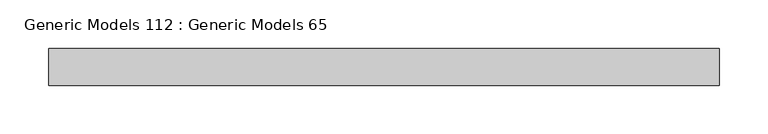
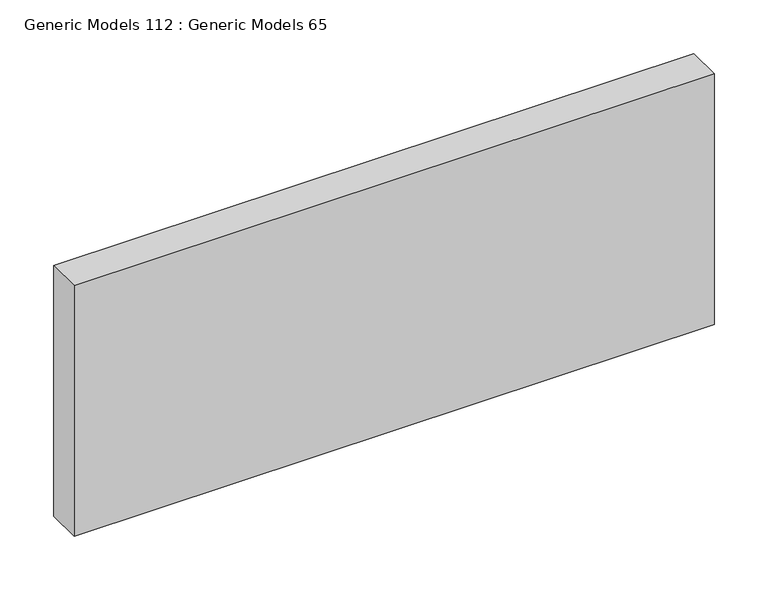
"""IFC4 building model written with IfcOpenShell, lengths in millimetres: proxy geometry, Generic Models 112 : Generic Models 65."""

import ifcopenshell
import ifcopenshell.guid

model = None  # the IFC model being written
_history = None  # IfcOwnerHistory: only IFC2X3 demands one
_inside = {}  # id of a spatial element -> (the spatial element, [elements in it])
_under = {}  # id of a project, library or spatial element -> (it, [spatial elements below it])
_declared = {}  # id of a project -> (the project, [libraries it declares])
_typed = {}  # id of a type object -> (the type object, [elements of that type])
_made_of = {}  # id of a material, layer set ... -> (it, [elements and type objects made of it])


def new_model(schema):
    """Start an empty IFC model of exactly this schema.

    Asked for "IFC4X3", IfcOpenShell would pick the latest addendum, in which some entities
    have other attributes; the version numbers below select the first issue.
    IFC2X3 requires an IfcOwnerHistory on every rooted entity: one is made here for all.
    """
    global model, _history
    if schema == "IFC4X3":
        model = ifcopenshell.file(schema_version=(4, 3, 0, 0))
    else:
        model = ifcopenshell.file(schema=schema)
    _inside.clear()
    _under.clear()
    _declared.clear()
    _typed.clear()
    _made_of.clear()
    _history = None
    if model.schema == "IFC2X3":
        org = make("IfcOrganization", Name="unknown")
        user = make(
            "IfcPersonAndOrganization",
            ThePerson=make("IfcPerson", FamilyName="unknown"),
            TheOrganization=org,
        )
        app = make(
            "IfcApplication",
            ApplicationDeveloper=org,
            Version="unknown",
            ApplicationFullName="unknown",
            ApplicationIdentifier="unknown",
        )
        _history = make(
            "IfcOwnerHistory",
            OwningUser=user,
            OwningApplication=app,
            ChangeAction="ADDED",
            CreationDate=0,
        )
    return model


def make(cls, **values):
    """One entity of the class cls with the attributes given. An attribute that is None is left unset."""
    return model.create_entity(
        cls, **{name: value for name, value in values.items() if value is not None}
    )


def rooted(cls, **values):
    """An entity with a GlobalId (a new one), such as an element, a storey or a relation."""
    return make(cls, GlobalId=ifcopenshell.guid.new(), OwnerHistory=_history, **values)


def si_unit(unit_type, name, prefix=None):
    """IfcSIUnit, for example si_unit("LENGTHUNIT", "METRE", prefix="MILLI")."""
    return make("IfcSIUnit", UnitType=unit_type, Prefix=prefix, Name=name)


def assignment(units):
    """IfcUnitAssignment: the units of a project."""
    return None if units is None else make("IfcUnitAssignment", Units=units)


def point(xyz):
    """IfcCartesianPoint."""
    return None if xyz is None else make("IfcCartesianPoint", Coordinates=xyz)


def direction(xyz):
    """IfcDirection."""
    return None if xyz is None else make("IfcDirection", DirectionRatios=xyz)


def frame(location, z_axis=None, x_axis=None):
    """IfcAxis2Placement3D, a coordinate frame: its origin and axes. An axis left out is left unset."""
    return make(
        "IfcAxis2Placement3D",
        Location=point(location),
        Axis=direction(z_axis),
        RefDirection=direction(x_axis),
    )


def origin():
    """The frame at (0, 0, 0) with its axes left unset."""
    return frame((0.0, 0.0, 0.0))


def place(relative_to, where):
    """IfcLocalPlacement: puts the frame where relative to a parent placement (None: the world)."""
    return make(
        "IfcLocalPlacement", PlacementRelTo=relative_to, RelativePlacement=where
    )


def context(
    kind, dimensions, precision=None, world=None, true_north=None, identifier=None
):
    """IfcGeometricRepresentationContext, for example the 3D "Model" context."""
    return make(
        "IfcGeometricRepresentationContext",
        ContextIdentifier=identifier,
        ContextType=kind,
        CoordinateSpaceDimension=dimensions,
        Precision=precision,
        WorldCoordinateSystem=world,
        TrueNorth=true_north,
    )


def project(units=None, contexts=None):
    """IfcProject with its units and contexts."""
    return rooted(
        "IfcProject",
        Name="project",
        RepresentationContexts=contexts,
        UnitsInContext=assignment(units),
    )


def spatial(cls, under=None, at=None, **own):
    """A site, building, storey or space (cls), placed at a placement, below another one or the project."""
    s = rooted(cls, ObjectPlacement=at, **own)
    if under is not None:
        _under.setdefault(under.id(), (under, []))[1].append(s)
    return s


def polyline(points):
    """IfcPolyline through the points."""
    return make("IfcPolyline", Points=[point(p) for p in points])


def outline(outer, holes=None, kind="AREA"):
    """IfcArbitraryClosedProfileDef: a profile drawn as a closed curve; with holes, ...WithVoids."""
    if holes is None:
        return make("IfcArbitraryClosedProfileDef", ProfileType=kind, OuterCurve=outer)
    return make(
        "IfcArbitraryProfileDefWithVoids",
        ProfileType=kind,
        OuterCurve=outer,
        InnerCurves=holes,
    )


def extrude(swept, where, along, depth):
    """IfcExtrudedAreaSolid: the profile swept, set in the frame where, extruded along a direction by depth."""
    return make(
        "IfcExtrudedAreaSolid",
        SweptArea=swept,
        Position=where,
        ExtrudedDirection=direction(along),
        Depth=depth,
    )


def shape(context_of_items, identifier, shape_type, items):
    """IfcShapeRepresentation: the items that make up one representation, for example the "Body"."""
    return make(
        "IfcShapeRepresentation",
        ContextOfItems=context_of_items,
        RepresentationIdentifier=identifier,
        RepresentationType=shape_type,
        Items=items,
    )


def source(mapping_origin, context_of_items, identifier, shape_type, items):
    """IfcRepresentationMap: a shape defined once, which mapped items show again and again."""
    return make(
        "IfcRepresentationMap",
        MappingOrigin=mapping_origin,
        MappedRepresentation=shape(context_of_items, identifier, shape_type, items),
    )


def transform(
    local_origin,
    x_axis=None,
    y_axis=None,
    z_axis=None,
    scale=None,
    scale2=None,
    scale3=None,
    uniform=True,
):
    """IfcCartesianTransformationOperator3D, or its non-uniform kind. x_axis, y_axis, z_axis: its Axis1, 2, 3."""
    if uniform:
        return make(
            "IfcCartesianTransformationOperator3D",
            Axis1=direction(x_axis),
            Axis2=direction(y_axis),
            LocalOrigin=point(local_origin),
            Scale=scale,
            Axis3=direction(z_axis),
        )
    return make(
        "IfcCartesianTransformationOperator3DnonUniform",
        Axis1=direction(x_axis),
        Axis2=direction(y_axis),
        LocalOrigin=point(local_origin),
        Scale=scale,
        Axis3=direction(z_axis),
        Scale2=scale2,
        Scale3=scale3,
    )


def mapped(mapping_source, mapping_target):
    """IfcMappedItem: shows the shape of a source again, moved by a transform."""
    return make(
        "IfcMappedItem", MappingSource=mapping_source, MappingTarget=mapping_target
    )


def made_of(thing, what):
    """Note that an element or type object is made of a material, layer set ...; save() writes the relation."""
    if what is not None:
        _made_of.setdefault(what.id(), (what, []))[1].append(thing)
    return thing


def element(
    cls,
    number,
    at=None,
    inside=None,
    cuts=None,
    type_object=None,
    material=None,
    context=None,
    identifier="Body",
    shape_type=None,
    held_by="IfcProductDefinitionShape",
    body=None,
    shapes=None,
    **own,
):
    """One element of the class cls, such as IfcWall. Its Tag is "e" and its number.

    at: its placement. inside: the storey or other place that contains it. cuts: it is an
    opening in that element (IfcRelVoidsElement). A single representation is given by context,
    identifier, shape_type and body (its items); several are given by shapes. held_by: the class
    of the entity that holds the representations. save() writes the other relations.
    """
    e = rooted(cls, Tag="e%d" % number, ObjectPlacement=at, **own)
    if body is not None:
        shapes = [shape(context, identifier, shape_type, body)]
    if shapes is not None:
        e.Representation = make(held_by, Representations=shapes)
    if inside is not None:
        _inside.setdefault(inside.id(), (inside, []))[1].append(e)
    if cuts is not None:
        rooted(
            "IfcRelVoidsElement", RelatingBuildingElement=cuts, RelatedOpeningElement=e
        )
    if type_object is not None:
        _typed.setdefault(type_object.id(), (type_object, []))[1].append(e)
    return made_of(e, material)


def aggregate(whole, parts):
    """IfcRelAggregates: a whole, such as a stair, and the parts it consists of."""
    return rooted("IfcRelAggregates", RelatingObject=whole, RelatedObjects=parts)


def save(model, path):
    """Write the relations noted so far, then the file.

    IfcRelAggregates (storeys below a building ...), IfcRelContainedInSpatialStructure (elements
    in a storey), IfcRelDefinesByType, IfcRelAssociatesMaterial and IfcRelDeclares: one each for
    every whole, place, type object, material and project.
    """
    for whole, parts in _under.values():
        aggregate(whole, parts)
    for where, things in _inside.values():
        rooted(
            "IfcRelContainedInSpatialStructure",
            RelatedElements=things,
            RelatingStructure=where,
        )
    for kind, things in _typed.values():
        rooted("IfcRelDefinesByType", RelatedObjects=things, RelatingType=kind)
    for what, things in _made_of.values():
        rooted("IfcRelAssociatesMaterial", RelatedObjects=things, RelatingMaterial=what)
    for by, libraries in _declared.values():
        rooted("IfcRelDeclares", RelatingContext=by, RelatedDefinitions=libraries)
    model.write(path)


def generic_models_112_generic_models_65_d168d7b0(model_context):
    return source(origin(), model_context, "Body", "SweptSolid", [
        extrude(outline(polyline([(50952.4, 592.1375), (50952.4, 630.2375), (51642.1451407, 630.2375), (51642.1451407, 592.1375), (50952.4, 592.1375)])), frame((0.0, 0.0, 5222.478125), z_axis=(0.0, 0.0, 1.0), x_axis=(1.0, 0.0, 0.0)), (0.0, 0.0, 1.0), 285.75),
    ])


if __name__ == "__main__":
    model = new_model("IFC4")
    model_context = context("Model", 3, world=origin())
    ifc_project = project(units=[si_unit("LENGTHUNIT", "METRE", prefix="MILLI")], contexts=[model_context])
    site = spatial("IfcSite", under=ifc_project)
    building = spatial("IfcBuilding", under=site)
    placement = place(None, origin())
    generic_models_112_generic_models_65_shape = generic_models_112_generic_models_65_d168d7b0(model_context)
    element("IfcBuildingElementProxy", 1, Name="Generic Models 112 : Generic Models 65", ObjectType="Generic Models 112 : Generic Models 65", at=placement, inside=building, context=model_context, shape_type="MappedRepresentation", body=[
        mapped(generic_models_112_generic_models_65_shape, transform((0.0, 0.0, 0.0), x_axis=(1.0, 0.0, 0.0), y_axis=(0.0, 1.0, 0.0), z_axis=(0.0, 0.0, 1.0))),
    ])
    save(model, "model.ifc")

# Revit data of these elements
# Element 1 (IfcBuildingElementProxy, "Generic Models 112 : Generic Models 65")
#   Materials on its faces: "WOOD JOIST AS SPECIFIED"
# Materials
#   "WOOD JOIST AS SPECIFIED": class "Wood", colour RGB 234 198 147, transparency 0, Description = "Pinus Echinata", Cost = 0
